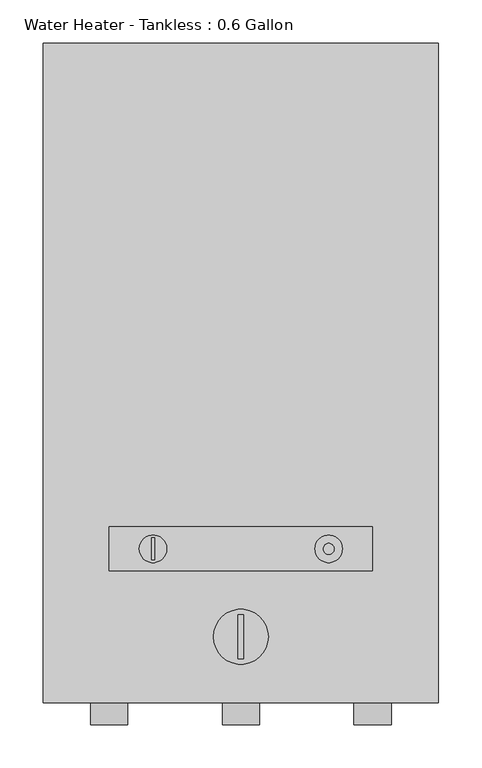
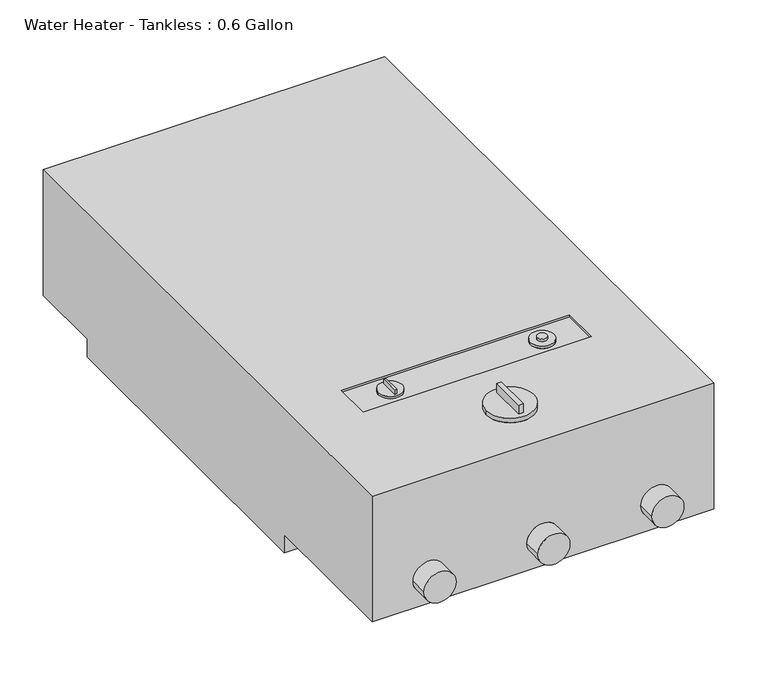
"""IFC4 building model written with IfcOpenShell, lengths in millimetres: proxy geometry, Water Heater - Tankless : 0.6 Gallon."""

import ifcopenshell
import ifcopenshell.guid

model = None  # the IFC model being written
_history = None  # IfcOwnerHistory: only IFC2X3 demands one
_inside = {}  # id of a spatial element -> (the spatial element, [elements in it])
_under = {}  # id of a project, library or spatial element -> (it, [spatial elements below it])
_declared = {}  # id of a project -> (the project, [libraries it declares])
_typed = {}  # id of a type object -> (the type object, [elements of that type])
_made_of = {}  # id of a material, layer set ... -> (it, [elements and type objects made of it])


def new_model(schema):
    """Start an empty IFC model of exactly this schema.

    Asked for "IFC4X3", IfcOpenShell would pick the latest addendum, in which some entities
    have other attributes; the version numbers below select the first issue.
    IFC2X3 requires an IfcOwnerHistory on every rooted entity: one is made here for all.
    """
    global model, _history
    if schema == "IFC4X3":
        model = ifcopenshell.file(schema_version=(4, 3, 0, 0))
    else:
        model = ifcopenshell.file(schema=schema)
    _inside.clear()
    _under.clear()
    _declared.clear()
    _typed.clear()
    _made_of.clear()
    _history = None
    if model.schema == "IFC2X3":
        org = make("IfcOrganization", Name="unknown")
        user = make(
            "IfcPersonAndOrganization",
            ThePerson=make("IfcPerson", FamilyName="unknown"),
            TheOrganization=org,
        )
        app = make(
            "IfcApplication",
            ApplicationDeveloper=org,
            Version="unknown",
            ApplicationFullName="unknown",
            ApplicationIdentifier="unknown",
        )
        _history = make(
            "IfcOwnerHistory",
            OwningUser=user,
            OwningApplication=app,
            ChangeAction="ADDED",
            CreationDate=0,
        )
    return model


def make(cls, **values):
    """One entity of the class cls with the attributes given. An attribute that is None is left unset."""
    return model.create_entity(
        cls, **{name: value for name, value in values.items() if value is not None}
    )


def rooted(cls, **values):
    """An entity with a GlobalId (a new one), such as an element, a storey or a relation."""
    return make(cls, GlobalId=ifcopenshell.guid.new(), OwnerHistory=_history, **values)


def si_unit(unit_type, name, prefix=None):
    """IfcSIUnit, for example si_unit("LENGTHUNIT", "METRE", prefix="MILLI")."""
    return make("IfcSIUnit", UnitType=unit_type, Prefix=prefix, Name=name)


def assignment(units):
    """IfcUnitAssignment: the units of a project."""
    return None if units is None else make("IfcUnitAssignment", Units=units)


def point(xyz):
    """IfcCartesianPoint."""
    return None if xyz is None else make("IfcCartesianPoint", Coordinates=xyz)


def direction(xyz):
    """IfcDirection."""
    return None if xyz is None else make("IfcDirection", DirectionRatios=xyz)


def frame(location, z_axis=None, x_axis=None):
    """IfcAxis2Placement3D, a coordinate frame: its origin and axes. An axis left out is left unset."""
    return make(
        "IfcAxis2Placement3D",
        Location=point(location),
        Axis=direction(z_axis),
        RefDirection=direction(x_axis),
    )


def frame_2d(location, x_axis=None):
    """IfcAxis2Placement2D, a coordinate frame in the plane: its origin and x axis."""
    return make(
        "IfcAxis2Placement2D", Location=point(location), RefDirection=direction(x_axis)
    )


def origin():
    """The frame at (0, 0, 0) with its axes left unset."""
    return frame((0.0, 0.0, 0.0))


def place(relative_to, where):
    """IfcLocalPlacement: puts the frame where relative to a parent placement (None: the world)."""
    return make(
        "IfcLocalPlacement", PlacementRelTo=relative_to, RelativePlacement=where
    )


def context(
    kind, dimensions, precision=None, world=None, true_north=None, identifier=None
):
    """IfcGeometricRepresentationContext, for example the 3D "Model" context."""
    return make(
        "IfcGeometricRepresentationContext",
        ContextIdentifier=identifier,
        ContextType=kind,
        CoordinateSpaceDimension=dimensions,
        Precision=precision,
        WorldCoordinateSystem=world,
        TrueNorth=true_north,
    )


def project(units=None, contexts=None):
    """IfcProject with its units and contexts."""
    return rooted(
        "IfcProject",
        Name="project",
        RepresentationContexts=contexts,
        UnitsInContext=assignment(units),
    )


def spatial(cls, under=None, at=None, **own):
    """A site, building, storey or space (cls), placed at a placement, below another one or the project."""
    s = rooted(cls, ObjectPlacement=at, **own)
    if under is not None:
        _under.setdefault(under.id(), (under, []))[1].append(s)
    return s


def circle_curve(where, radius):
    """IfcCircle in the frame where."""
    return make("IfcCircle", Position=where, Radius=radius)


def trimmed(basis, trim1, trim2, sense, master):
    """IfcTrimmedCurve: the piece of a basis curve between two trims."""
    return make(
        "IfcTrimmedCurve",
        BasisCurve=basis,
        Trim1=trim1,
        Trim2=trim2,
        SenseAgreement=sense,
        MasterRepresentation=master,
    )


def segment(curve, same_sense, transition):
    """IfcCompositeCurveSegment."""
    return make(
        "IfcCompositeCurveSegment",
        Transition=transition,
        SameSense=same_sense,
        ParentCurve=curve,
    )


def composite_curve(segments, self_intersect=None):
    """IfcCompositeCurve: segments joined end to end."""
    return make("IfcCompositeCurve", Segments=segments, SelfIntersect=self_intersect)


def outline(outer, holes=None, kind="AREA"):
    """IfcArbitraryClosedProfileDef: a profile drawn as a closed curve; with holes, ...WithVoids."""
    if holes is None:
        return make("IfcArbitraryClosedProfileDef", ProfileType=kind, OuterCurve=outer)
    return make(
        "IfcArbitraryProfileDefWithVoids",
        ProfileType=kind,
        OuterCurve=outer,
        InnerCurves=holes,
    )


def extrude(swept, where, along, depth):
    """IfcExtrudedAreaSolid: the profile swept, set in the frame where, extruded along a direction by depth."""
    return make(
        "IfcExtrudedAreaSolid",
        SweptArea=swept,
        Position=where,
        ExtrudedDirection=direction(along),
        Depth=depth,
    )


def shape(context_of_items, identifier, shape_type, items):
    """IfcShapeRepresentation: the items that make up one representation, for example the "Body"."""
    return make(
        "IfcShapeRepresentation",
        ContextOfItems=context_of_items,
        RepresentationIdentifier=identifier,
        RepresentationType=shape_type,
        Items=items,
    )


def source(mapping_origin, context_of_items, identifier, shape_type, items):
    """IfcRepresentationMap: a shape defined once, which mapped items show again and again."""
    return make(
        "IfcRepresentationMap",
        MappingOrigin=mapping_origin,
        MappedRepresentation=shape(context_of_items, identifier, shape_type, items),
    )


def transform(
    local_origin,
    x_axis=None,
    y_axis=None,
    z_axis=None,
    scale=None,
    scale2=None,
    scale3=None,
    uniform=True,
):
    """IfcCartesianTransformationOperator3D, or its non-uniform kind. x_axis, y_axis, z_axis: its Axis1, 2, 3."""
    if uniform:
        return make(
            "IfcCartesianTransformationOperator3D",
            Axis1=direction(x_axis),
            Axis2=direction(y_axis),
            LocalOrigin=point(local_origin),
            Scale=scale,
            Axis3=direction(z_axis),
        )
    return make(
        "IfcCartesianTransformationOperator3DnonUniform",
        Axis1=direction(x_axis),
        Axis2=direction(y_axis),
        LocalOrigin=point(local_origin),
        Scale=scale,
        Axis3=direction(z_axis),
        Scale2=scale2,
        Scale3=scale3,
    )


def mapped(mapping_source, mapping_target):
    """IfcMappedItem: shows the shape of a source again, moved by a transform."""
    return make(
        "IfcMappedItem", MappingSource=mapping_source, MappingTarget=mapping_target
    )


def made_of(thing, what):
    """Note that an element or type object is made of a material, layer set ...; save() writes the relation."""
    if what is not None:
        _made_of.setdefault(what.id(), (what, []))[1].append(thing)
    return thing


def element(
    cls,
    number,
    at=None,
    inside=None,
    cuts=None,
    type_object=None,
    material=None,
    context=None,
    identifier="Body",
    shape_type=None,
    held_by="IfcProductDefinitionShape",
    body=None,
    shapes=None,
    **own,
):
    """One element of the class cls, such as IfcWall. Its Tag is "e" and its number.

    at: its placement. inside: the storey or other place that contains it. cuts: it is an
    opening in that element (IfcRelVoidsElement). A single representation is given by context,
    identifier, shape_type and body (its items); several are given by shapes. held_by: the class
    of the entity that holds the representations. save() writes the other relations.
    """
    e = rooted(cls, Tag="e%d" % number, ObjectPlacement=at, **own)
    if body is not None:
        shapes = [shape(context, identifier, shape_type, body)]
    if shapes is not None:
        e.Representation = make(held_by, Representations=shapes)
    if inside is not None:
        _inside.setdefault(inside.id(), (inside, []))[1].append(e)
    if cuts is not None:
        rooted(
            "IfcRelVoidsElement", RelatingBuildingElement=cuts, RelatedOpeningElement=e
        )
    if type_object is not None:
        _typed.setdefault(type_object.id(), (type_object, []))[1].append(e)
    return made_of(e, material)


def aggregate(whole, parts):
    """IfcRelAggregates: a whole, such as a stair, and the parts it consists of."""
    return rooted("IfcRelAggregates", RelatingObject=whole, RelatedObjects=parts)


def save(model, path):
    """Write the relations noted so far, then the file.

    IfcRelAggregates (storeys below a building ...), IfcRelContainedInSpatialStructure (elements
    in a storey), IfcRelDefinesByType, IfcRelAssociatesMaterial and IfcRelDeclares: one each for
    every whole, place, type object, material and project.
    """
    for whole, parts in _under.values():
        aggregate(whole, parts)
    for where, things in _inside.values():
        rooted(
            "IfcRelContainedInSpatialStructure",
            RelatedElements=things,
            RelatingStructure=where,
        )
    for kind, things in _typed.values():
        rooted("IfcRelDefinesByType", RelatedObjects=things, RelatingType=kind)
    for what, things in _made_of.values():
        rooted("IfcRelAssociatesMaterial", RelatedObjects=things, RelatingMaterial=what)
    for by, libraries in _declared.values():
        rooted("IfcRelDeclares", RelatingContext=by, RelatedDefinitions=libraries)
    model.write(path)


def plane_surface(at):
    """IfcPlane: the flat surface through the origin of the frame at, square to its z axis."""
    return make("IfcPlane", Position=at)


def cylinder_surface(at, radius):
    """IfcCylindricalSurface: all points at the distance radius from the z axis of the frame at."""
    return make("IfcCylindricalSurface", Position=at, Radius=radius)


def advanced_brep(points, edges, surfaces, faces):
    """IfcAdvancedBrep: a solid bounded by faces that lie on surfaces and meet in shared edges.

    An edge is (start, end): straight between two places in points (the first is 0);
    or (start, end, curve); or (start, end, curve, False) where it runs against its curve.
    A face is (place in surfaces, loops), or (place, loops, False) where it looks against
    its surface's normal. A loop lists edges by number (the first is 1), with a minus sign
    where the edge is run from its end to its start. The first loop is the outer one.
    """
    corners = [point(p) for p in points]
    vertices = [make("IfcVertexPoint", VertexGeometry=c) for c in corners]
    made = []
    for start, end, *more in edges:
        made.append(
            make(
                "IfcEdgeCurve",
                EdgeStart=vertices[start],
                EdgeEnd=vertices[end],
                EdgeGeometry=more[0] if more else make("IfcPolyline", Points=[corners[start], corners[end]]),
                SameSense=more[1] if len(more) > 1 else True,
            )
        )
    hull = []
    for where, loops, *sense in faces:
        bounds = []
        for j, loop in enumerate(loops):
            ring = [make("IfcOrientedEdge", EdgeElement=made[abs(k) - 1], Orientation=k > 0) for k in loop]
            bounds.append(
                make(
                    "IfcFaceOuterBound" if j == 0 else "IfcFaceBound",
                    Bound=make("IfcEdgeLoop", EdgeList=ring),
                    Orientation=True,
                )
            )
        hull.append(make("IfcAdvancedFace", Bounds=bounds, FaceSurface=surfaces[where], SameSense=sense[0] if sense else True))
    return make("IfcAdvancedBrep", Outer=make("IfcClosedShell", CfsFaces=hull))


def water_heater_tankless_0_6_gallon_c20ab9af(model_context):
    return source(origin(), model_context, "Body", "SolidModel", [
        advanced_brep(
        [(228.6, 762.0, 25.4), (228.6, 762.0, 203.2), (228.6, 0.0, 203.2), (228.6, 0.0, 25.4), (228.6, 203.2, 25.4), (228.6, 203.2, 0.0), (228.6, 660.4, 0.0), (228.6, 660.4, 25.4), (-228.6, 762.0, 25.4), (-228.6, 660.4, 25.4), (-228.6, 660.4, 0.0), (-228.6, 203.2, 0.0), (-228.6, 203.2, 25.4), (-228.6, 0.0, 25.4), (-228.6, 0.0, 203.2), (-228.6, 762.0, 203.2), (-152.4, 203.2, 203.2), (152.4, 203.2, 203.2), (152.4, 152.4, 203.2), (-152.4, 152.4, 203.2), (31.75, 76.2, 203.2), (-31.75, 76.2, 203.2), (-130.96875, 0.0, 63.5), (-173.83125, 0.0, 63.5), (21.43125, 0.0, 63.5), (-21.43125, 0.0, 63.5), (173.83125, 0.0, 63.5), (130.96875, 0.0, 63.5), (152.4, 203.2, 200.025), (-152.4, 203.2, 200.025), (-152.4, 152.4, 200.025), (152.4, 152.4, 200.025), (-85.725, 177.8, 200.025), (-117.475, 177.8, 200.025), (117.475, 177.8, 200.025), (85.725, 177.8, 200.025), (-173.83125, -25.4, 63.5), (-130.96875, -25.4, 63.5), (-21.43125, -25.4, 63.5), (21.43125, -25.4, 63.5), (130.96875, -25.4, 63.5), (173.83125, -25.4, 63.5), (-117.475, 177.8, 203.2), (-85.725, 177.8, 203.2), (-103.1875, 190.5, 203.2), (-100.0125, 190.5, 203.2), (-100.0125, 165.1, 203.2), (-103.1875, 165.1, 203.2), (85.725, 177.8, 203.2), (117.475, 177.8, 203.2), (107.95, 177.8, 203.2), (95.25, 177.8, 203.2), (95.25, 177.8, 206.375), (107.95, 177.8, 206.375), (-100.0125, 190.5, 209.55), (-103.1875, 190.5, 209.55), (-103.1875, 165.1, 209.55), (-100.0125, 165.1, 209.55), (-31.75, 76.2, 209.55), (31.75, 76.2, 209.55), (-3.175, 101.6, 209.55), (3.175, 101.6, 209.55), (3.175, 50.8, 209.55), (-3.175, 50.8, 209.55), (3.175, 101.6, 222.25), (-3.175, 101.6, 222.25), (-3.175, 50.8, 222.25), (3.175, 50.8, 222.25)],
        [
            (0, 1),
            (1, 2),
            (2, 3),
            (3, 4),
            (4, 5),
            (5, 6),
            (6, 7),
            (7, 0),
            (8, 9),
            (9, 10),
            (10, 11),
            (11, 12),
            (12, 13),
            (13, 14),
            (14, 15),
            (15, 8),
            (0, 8),
            (15, 1),
            (14, 2),
            (16, 17),
            (17, 18),
            (18, 19),
            (19, 16),
            (20, 21, circle_curve(frame((0.0, 76.2, 203.2), z_axis=(0.0, 0.0, -1.0), x_axis=(1.0, 0.0, 0.0)), 31.75)),
            (21, 20, circle_curve(frame((0.0, 76.2, 203.2), z_axis=(0.0, 0.0, -1.0), x_axis=(1.0, 0.0, 0.0)), 31.75)),
            (13, 3),
            (22, 23, circle_curve(frame((-152.4, 0.0, 63.5), z_axis=(0.0, 1.0, 0.0), x_axis=(1.0, 0.0, 0.0)), 21.43125)),
            (23, 22, circle_curve(frame((-152.4, 0.0, 63.5), z_axis=(0.0, 1.0, 0.0), x_axis=(1.0, 0.0, 0.0)), 21.43125)),
            (24, 25, circle_curve(frame((0.0, 0.0, 63.5), z_axis=(0.0, 1.0, 0.0), x_axis=(1.0, 0.0, 0.0)), 21.43125)),
            (25, 24, circle_curve(frame((0.0, 0.0, 63.5), z_axis=(0.0, 1.0, 0.0), x_axis=(1.0, 0.0, 0.0)), 21.43125)),
            (26, 27, circle_curve(frame((152.4, 0.0, 63.5), z_axis=(0.0, 1.0, 0.0), x_axis=(1.0, 0.0, 0.0)), 21.43125)),
            (27, 26, circle_curve(frame((152.4, 0.0, 63.5), z_axis=(0.0, 1.0, 0.0), x_axis=(1.0, 0.0, 0.0)), 21.43125)),
            (12, 4),
            (11, 5),
            (10, 6),
            (9, 7),
            (28, 29),
            (29, 30),
            (30, 31),
            (31, 28),
            (32, 33, circle_curve(frame((-101.6, 177.8, 200.025), z_axis=(0.0, 0.0, -1.0), x_axis=(1.0, 0.0, 0.0)), 15.875)),
            (33, 32, circle_curve(frame((-101.6, 177.8, 200.025), z_axis=(0.0, 0.0, -1.0), x_axis=(1.0, 0.0, 0.0)), 15.875)),
            (34, 35, circle_curve(frame((101.6, 177.8, 200.025), z_axis=(0.0, 0.0, -1.0), x_axis=(1.0, 0.0, 0.0)), 15.875)),
            (35, 34, circle_curve(frame((101.6, 177.8, 200.025), z_axis=(0.0, 0.0, -1.0), x_axis=(1.0, 0.0, 0.0)), 15.875)),
            (28, 17),
            (16, 29),
            (19, 30),
            (18, 31),
            (36, 37, circle_curve(frame((-152.4, -25.4, 63.5), z_axis=(0.0, -1.0, 0.0), x_axis=(1.0, 0.0, 0.0)), 21.43125)),
            (37, 36, circle_curve(frame((-152.4, -25.4, 63.5), z_axis=(0.0, -1.0, 0.0), x_axis=(1.0, 0.0, 0.0)), 21.43125)),
            (38, 39, circle_curve(frame((0.0, -25.4, 63.5), z_axis=(0.0, -1.0, 0.0), x_axis=(1.0, 0.0, 0.0)), 21.43125)),
            (39, 38, circle_curve(frame((0.0, -25.4, 63.5), z_axis=(0.0, -1.0, 0.0), x_axis=(1.0, 0.0, 0.0)), 21.43125)),
            (40, 41, circle_curve(frame((152.4, -25.4, 63.5), z_axis=(0.0, -1.0, 0.0), x_axis=(1.0, 0.0, 0.0)), 21.43125)),
            (41, 40, circle_curve(frame((152.4, -25.4, 63.5), z_axis=(0.0, -1.0, 0.0), x_axis=(1.0, 0.0, 0.0)), 21.43125)),
            (36, 23),
            (22, 37),
            (38, 25),
            (24, 39),
            (40, 27),
            (26, 41),
            (42, 43, circle_curve(frame((-101.6, 177.8, 203.2), z_axis=(0.0, 0.0, 1.0), x_axis=(1.0, 0.0, 0.0)), 15.875)),
            (43, 42, circle_curve(frame((-101.6, 177.8, 203.2), z_axis=(0.0, 0.0, 1.0), x_axis=(1.0, 0.0, 0.0)), 15.875)),
            (44, 45),
            (45, 46),
            (46, 47),
            (47, 44),
            (48, 49, circle_curve(frame((101.6, 177.8, 203.2), z_axis=(0.0, 0.0, 1.0), x_axis=(1.0, 0.0, 0.0)), 15.875)),
            (49, 48, circle_curve(frame((101.6, 177.8, 203.2), z_axis=(0.0, 0.0, 1.0), x_axis=(1.0, 0.0, 0.0)), 15.875)),
            (50, 51, circle_curve(frame((101.6, 177.8, 203.2), z_axis=(0.0, 0.0, -1.0), x_axis=(1.0, 0.0, 0.0)), 6.35)),
            (51, 50, circle_curve(frame((101.6, 177.8, 203.2), z_axis=(0.0, 0.0, -1.0), x_axis=(1.0, 0.0, 0.0)), 6.35)),
            (42, 33),
            (32, 43),
            (48, 35),
            (34, 49),
            (52, 53, circle_curve(frame((101.6, 177.8, 206.375), z_axis=(0.0, 0.0, 1.0), x_axis=(1.0, 0.0, 0.0)), 6.35)),
            (53, 52, circle_curve(frame((101.6, 177.8, 206.375), z_axis=(0.0, 0.0, 1.0), x_axis=(1.0, 0.0, 0.0)), 6.35)),
            (52, 51),
            (50, 53),
            (54, 55),
            (55, 56),
            (56, 57),
            (57, 54),
            (54, 45),
            (44, 55),
            (47, 56),
            (46, 57),
            (58, 59, circle_curve(frame((0.0, 76.2, 209.55), z_axis=(0.0, 0.0, 1.0), x_axis=(1.0, 0.0, 0.0)), 31.75)),
            (59, 58, circle_curve(frame((0.0, 76.2, 209.55), z_axis=(0.0, 0.0, 1.0), x_axis=(1.0, 0.0, 0.0)), 31.75)),
            (60, 61),
            (61, 62),
            (62, 63),
            (63, 60),
            (58, 21),
            (20, 59),
            (64, 65),
            (65, 66),
            (66, 67),
            (67, 64),
            (64, 61),
            (60, 65),
            (63, 66),
            (62, 67),
        ],
        [
            plane_surface(frame((228.6, 762.0, 203.2), z_axis=(1.0, 0.0, 0.0), x_axis=(0.0, 0.0, 1.0))),
            plane_surface(frame((-228.6, 762.0, 203.2), z_axis=(-1.0, 0.0, 0.0), x_axis=(0.0, 0.0, -1.0))),
            plane_surface(frame((228.6, 762.0, 25.4), z_axis=(0.0, 1.0, 0.0), x_axis=(-1.0, 0.0, 0.0))),
            plane_surface(frame((228.6, 762.0, 203.2), z_axis=(0.0, 0.0, 1.0), x_axis=(-1.0, 0.0, 0.0))),
            plane_surface(frame((228.6, 0.0, 203.2), z_axis=(0.0, -1.0, 0.0), x_axis=(-1.0, 0.0, 0.0))),
            plane_surface(frame((228.6, 0.0, 25.4), z_axis=(0.0, 0.0, -1.0), x_axis=(-1.0, 0.0, 0.0))),
            plane_surface(frame((228.6, 203.2, 25.4), z_axis=(0.0, -1.0, 0.0), x_axis=(-1.0, 0.0, 0.0))),
            plane_surface(frame((228.6, 203.2, 0.0), z_axis=(0.0, 0.0, -1.0), x_axis=(-1.0, 0.0, 0.0))),
            plane_surface(frame((228.6, 660.4, 0.0), z_axis=(0.0, 1.0, 0.0), x_axis=(-1.0, 0.0, 0.0))),
            plane_surface(frame((228.6, 660.4, 25.4), z_axis=(0.0, 0.0, -1.0), x_axis=(-1.0, 0.0, 0.0))),
            plane_surface(frame((-152.4, 203.2, 200.025), z_axis=(0.0, 0.0, 1.0), x_axis=(1.0, 0.0, 0.0))),
            plane_surface(frame((152.4, 203.2, 203.2), z_axis=(0.0, -1.0, 0.0), x_axis=(0.0, 0.0, -1.0))),
            plane_surface(frame((-152.4, 203.2, 203.2), z_axis=(1.0, 0.0, 0.0), x_axis=(0.0, 0.0, -1.0))),
            plane_surface(frame((-152.4, 152.4, 203.2), z_axis=(0.0, 1.0, 0.0), x_axis=(0.0, 0.0, -1.0))),
            plane_surface(frame((152.4, 152.4, 203.2), z_axis=(-1.0, 0.0, 0.0), x_axis=(0.0, 0.0, -1.0))),
            plane_surface(frame((-130.96875, -25.4, 63.5), z_axis=(0.0, -1.0, 0.0), x_axis=(0.0, 0.0, 1.0))),
            cylinder_surface(frame((-152.4, 0.0, 63.5), z_axis=(0.0, -1.0, 0.0), x_axis=(1.0, 0.0, 0.0)), 21.43125),
            cylinder_surface(frame((0.0, 0.0, 63.5), z_axis=(0.0, -1.0, 0.0), x_axis=(1.0, 0.0, 0.0)), 21.43125),
            cylinder_surface(frame((152.4, 0.0, 63.5), z_axis=(0.0, -1.0, 0.0), x_axis=(1.0, 0.0, 0.0)), 21.43125),
            plane_surface(frame((-85.725, 177.8, 203.2), z_axis=(0.0, 0.0, 1.0), x_axis=(0.0, 1.0, 0.0))),
            cylinder_surface(frame((-101.6, 177.8, 200.025), z_axis=(0.0, 0.0, 1.0), x_axis=(1.0, 0.0, 0.0)), 15.875),
            cylinder_surface(frame((101.6, 177.8, 0.0), z_axis=(0.0, 0.0, 1.0), x_axis=(1.0, 0.0, 0.0)), 15.875),
            plane_surface(frame((107.95, 177.8, 206.375), z_axis=(0.0, 0.0, 1.0), x_axis=(0.0, 1.0, 0.0))),
            cylinder_surface(frame((101.6, 177.8, 203.2), z_axis=(0.0, 0.0, 1.0), x_axis=(1.0, 0.0, 0.0)), 6.35),
            plane_surface(frame((-103.1875, 190.5, 209.55), z_axis=(0.0, 0.0, 1.0), x_axis=(-1.0, 0.0, 0.0))),
            plane_surface(frame((-100.0125, 190.5, 209.55), z_axis=(0.0, 1.0, 0.0), x_axis=(0.0, 0.0, -1.0))),
            plane_surface(frame((-103.1875, 190.5, 209.55), z_axis=(-1.0, 0.0, 0.0), x_axis=(0.0, 0.0, -1.0))),
            plane_surface(frame((-103.1875, 165.1, 209.55), z_axis=(0.0, -1.0, 0.0), x_axis=(0.0, 0.0, -1.0))),
            plane_surface(frame((-100.0125, 165.1, 209.55), z_axis=(1.0, 0.0, 0.0), x_axis=(0.0, 0.0, -1.0))),
            plane_surface(frame((31.75, 76.2, 209.55), z_axis=(0.0, 0.0, 1.0), x_axis=(0.0, 1.0, 0.0))),
            cylinder_surface(frame((0.0, 76.2, 203.2), z_axis=(0.0, 0.0, 1.0), x_axis=(1.0, 0.0, 0.0)), 31.75),
            plane_surface(frame((-3.175, 101.6, 222.25), z_axis=(0.0, 0.0, 1.0), x_axis=(-1.0, 0.0, 0.0))),
            plane_surface(frame((3.175, 101.6, 222.25), z_axis=(0.0, 1.0, 0.0), x_axis=(0.0, 0.0, -1.0))),
            plane_surface(frame((-3.175, 101.6, 222.25), z_axis=(-1.0, 0.0, 0.0), x_axis=(0.0, 0.0, -1.0))),
            plane_surface(frame((-3.175, 50.8, 222.25), z_axis=(0.0, -1.0, 0.0), x_axis=(0.0, 0.0, -1.0))),
            plane_surface(frame((3.175, 50.8, 222.25), z_axis=(1.0, 0.0, 0.0), x_axis=(0.0, 0.0, -1.0))),
        ],
        [
            (0, [[1, 2, 3, 4, 5, 6, 7, 8]]),
            (1, [[9, 10, 11, 12, 13, 14, 15, 16]]),
            (2, [[-1, 17, -16, 18]]),
            (3, [[-2, -18, -15, 19], [20, 21, 22, 23], [24, 25]]),
            (4, [[-3, -19, -14, 26], [27, 28], [29, 30], [31, 32]]),
            (5, [[-4, -26, -13, 33]]),
            (6, [[-5, -33, -12, 34]]),
            (7, [[-6, -34, -11, 35]]),
            (8, [[-7, -35, -10, 36]]),
            (9, [[-8, -36, -9, -17]]),
            (10, [[37, 38, 39, 40], [41, 42], [43, 44]]),
            (11, [[-37, 45, -20, 46]]),
            (12, [[-38, -46, -23, 47]]),
            (13, [[-39, -47, -22, 48]]),
            (14, [[-40, -48, -21, -45]]),
            (15, [[49, 50]]),
            (15, [[51, 52]]),
            (15, [[53, 54]]),
            (16, [[-49, 55, -27, 56]]),
            (16, [[-50, -56, -28, -55]]),
            (17, [[-51, 57, -29, 58]]),
            (17, [[-52, -58, -30, -57]]),
            (18, [[-53, 59, -31, 60]]),
            (18, [[-54, -60, -32, -59]]),
            (19, [[61, 62], [63, 64, 65, 66]]),
            (19, [[67, 68], [69, 70]]),
            (20, [[-61, 71, -41, 72]]),
            (20, [[-62, -72, -42, -71]]),
            (21, [[-67, 73, -43, 74]]),
            (21, [[-68, -74, -44, -73]]),
            (22, [[75, 76]]),
            (23, [[-75, 77, -69, 78]]),
            (23, [[-76, -78, -70, -77]]),
            (24, [[79, 80, 81, 82]]),
            (25, [[-79, 83, -63, 84]]),
            (26, [[-80, -84, -66, 85]]),
            (27, [[-81, -85, -65, 86]]),
            (28, [[-82, -86, -64, -83]]),
            (29, [[87, 88], [89, 90, 91, 92]]),
            (30, [[-87, 93, -24, 94]]),
            (30, [[-88, -94, -25, -93]]),
            (31, [[95, 96, 97, 98]]),
            (32, [[-95, 99, -89, 100]]),
            (33, [[-96, -100, -92, 101]]),
            (34, [[-97, -101, -91, 102]]),
            (35, [[-98, -102, -90, -99]]),
        ],
    ),
        extrude(outline(composite_curve([segment(trimmed(circle_curve(frame_2d((0.0, 152.4)), 3.175), [point((-3.175, 152.4))], [point((3.175, 152.4))], False, "CARTESIAN"), True, "CONTINUOUS"), segment(trimmed(circle_curve(frame_2d((0.0, 152.4)), 3.175), [point((3.175, 152.4))], [point((-3.175, 152.4))], False, "CARTESIAN"), True, "CONTINUOUS")], self_intersect=False)), frame((0.0, 0.0, 25.4), z_axis=(0.0, 0.0, 1.0), x_axis=(1.0, 0.0, 0.0)), (0.0, 0.0, 1.0), 38.1),
    ])


if __name__ == "__main__":
    model = new_model("IFC4")
    model_context = context("Model", 3, world=origin())
    ifc_project = project(units=[si_unit("LENGTHUNIT", "METRE", prefix="MILLI")], contexts=[model_context])
    site = spatial("IfcSite", under=ifc_project)
    building = spatial("IfcBuilding", under=site)
    placement = place(None, origin())
    water_heater_tankless_0_6_gallon_shape = water_heater_tankless_0_6_gallon_c20ab9af(model_context)
    element("IfcBuildingElementProxy", 1, Name="Water Heater - Tankless : 0.6 Gallon", ObjectType="Water Heater - Tankless : 0.6 Gallon", at=placement, inside=building, context=model_context, shape_type="MappedRepresentation", body=[
        mapped(water_heater_tankless_0_6_gallon_shape, transform((0.0, 0.0, 0.0), x_axis=(1.0, 0.0, 0.0), y_axis=(0.0, 1.0, 0.0), z_axis=(0.0, 0.0, 1.0))),
    ])
    save(model, "model.ifc")

# Revit data of these elements
# Type "Water Heater - Tankless : 0.6 Gallon"
#   Water Heater Width = 203.2 mm
#   Water Heater Length = 457.2 mm
#   Water Heater Height = 762 mm
#   Voltage = 120 V
#   Vent Radius = 2"
#   Vent Diameter = 4"
#   Hot Water Radius = 1/2"
#   Hot Water Diameter = 1"
#   Half Water Heater Length = 228.6 mm
#   Gas Radius = 3/8"
#   Gas Diameter = 3/4"
#   Flow Pressure [instance default] = 25.00 psi
#   Flow [instance default] = 13 GPM
#   Default Elevation = 1524 mm
#   Cold Water Radius = 1/2"
#   Cold Water Diameter = 1"
#   Apparent Load = 125 VA
#   Number of Poles = 1
#   Water Heater Material = none
#   Load Classification = Appliance - Dwelling Unit
# Element 1 (IfcBuildingElementProxy, "Water Heater - Tankless : 0.6 Gallon")
#   Flow = 0 GPM
